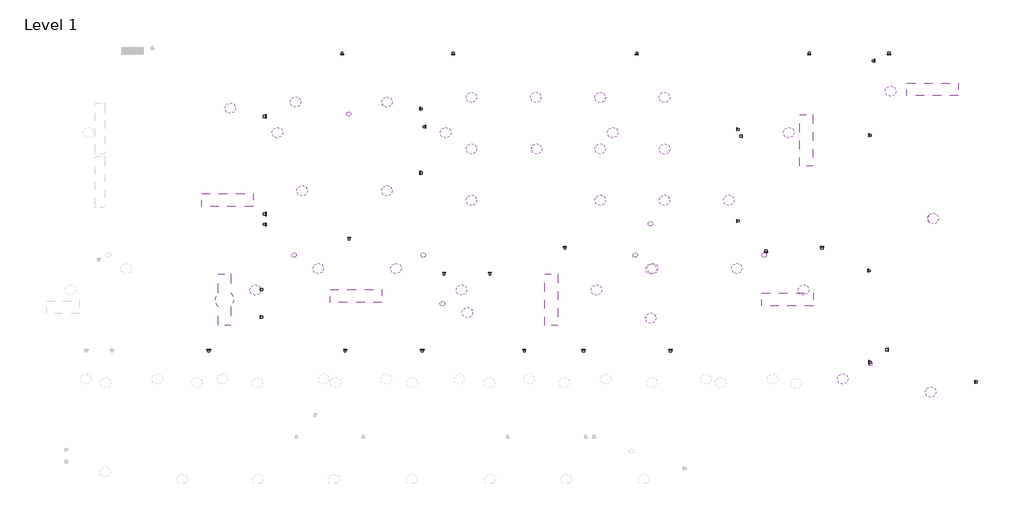
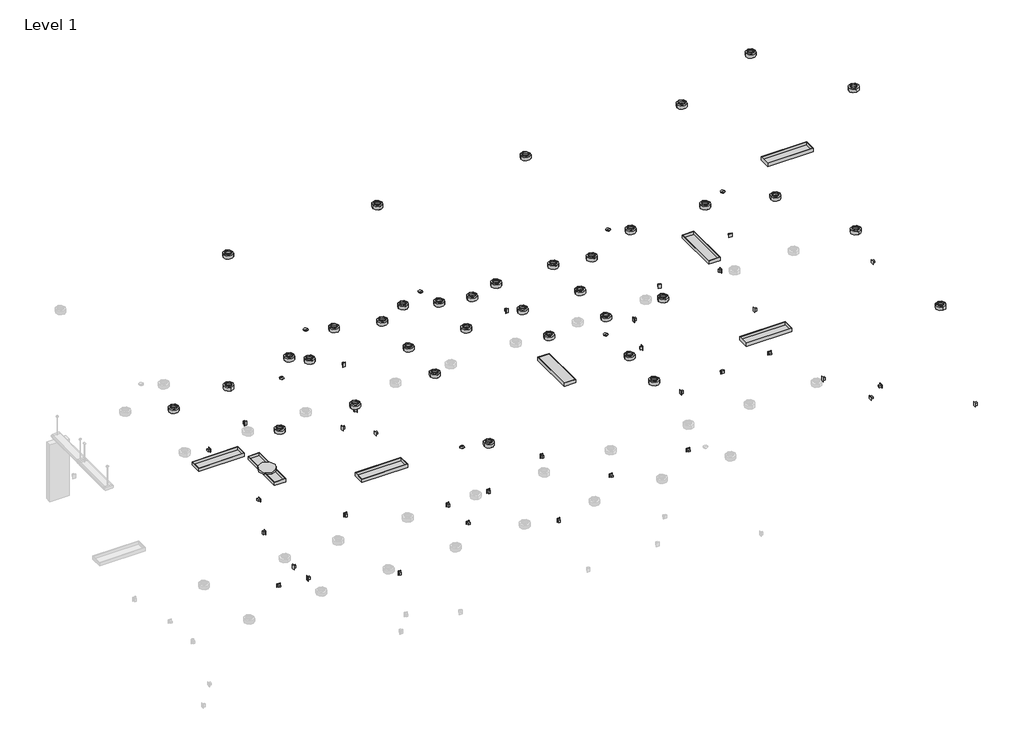
# One storey, part 3 of 3: 43 light fixtures, 22 proxies, 20 switching devices.
"""IFC4 building model written with IfcOpenShell, lengths in millimetres."""

import ifcopenshell
import ifcopenshell.guid

model = None  # the IFC model being written
_history = None  # IfcOwnerHistory: only IFC2X3 demands one
_inside = {}  # id of a spatial element -> (the spatial element, [elements in it])
_under = {}  # id of a project, library or spatial element -> (it, [spatial elements below it])
_declared = {}  # id of a project -> (the project, [libraries it declares])
_typed = {}  # id of a type object -> (the type object, [elements of that type])
_made_of = {}  # id of a material, layer set ... -> (it, [elements and type objects made of it])


def new_model(schema):
    """Start an empty IFC model of exactly this schema.

    Asked for "IFC4X3", IfcOpenShell would pick the latest addendum, in which some entities
    have other attributes; the version numbers below select the first issue.
    IFC2X3 requires an IfcOwnerHistory on every rooted entity: one is made here for all.
    """
    global model, _history
    if schema == "IFC4X3":
        model = ifcopenshell.file(schema_version=(4, 3, 0, 0))
    else:
        model = ifcopenshell.file(schema=schema)
    _inside.clear()
    _under.clear()
    _declared.clear()
    _typed.clear()
    _made_of.clear()
    _history = None
    if model.schema == "IFC2X3":
        org = make("IfcOrganization", Name="unknown")
        user = make(
            "IfcPersonAndOrganization",
            ThePerson=make("IfcPerson", FamilyName="unknown"),
            TheOrganization=org,
        )
        app = make(
            "IfcApplication",
            ApplicationDeveloper=org,
            Version="unknown",
            ApplicationFullName="unknown",
            ApplicationIdentifier="unknown",
        )
        _history = make(
            "IfcOwnerHistory",
            OwningUser=user,
            OwningApplication=app,
            ChangeAction="ADDED",
            CreationDate=0,
        )
    return model


def make(cls, **values):
    """One entity of the class cls with the attributes given. An attribute that is None is left unset."""
    return model.create_entity(
        cls, **{name: value for name, value in values.items() if value is not None}
    )


def rooted(cls, **values):
    """An entity with a GlobalId (a new one), such as an element, a storey or a relation."""
    return make(cls, GlobalId=ifcopenshell.guid.new(), OwnerHistory=_history, **values)


def si_unit(unit_type, name, prefix=None):
    """IfcSIUnit, for example si_unit("LENGTHUNIT", "METRE", prefix="MILLI")."""
    return make("IfcSIUnit", UnitType=unit_type, Prefix=prefix, Name=name)


def assignment(units):
    """IfcUnitAssignment: the units of a project."""
    return None if units is None else make("IfcUnitAssignment", Units=units)


def point(xyz):
    """IfcCartesianPoint."""
    return None if xyz is None else make("IfcCartesianPoint", Coordinates=xyz)


def direction(xyz):
    """IfcDirection."""
    return None if xyz is None else make("IfcDirection", DirectionRatios=xyz)


def frame(location, z_axis=None, x_axis=None):
    """IfcAxis2Placement3D, a coordinate frame: its origin and axes. An axis left out is left unset."""
    return make(
        "IfcAxis2Placement3D",
        Location=point(location),
        Axis=direction(z_axis),
        RefDirection=direction(x_axis),
    )


def frame_2d(location, x_axis=None):
    """IfcAxis2Placement2D, a coordinate frame in the plane: its origin and x axis."""
    return make(
        "IfcAxis2Placement2D", Location=point(location), RefDirection=direction(x_axis)
    )


def origin():
    """The frame at (0, 0, 0) with its axes left unset."""
    return frame((0.0, 0.0, 0.0))


def origin_with_axes():
    """The frame at (0, 0, 0) with the z axis (0, 0, 1) and the x axis (1, 0, 0) written out."""
    return frame((0.0, 0.0, 0.0), z_axis=(0.0, 0.0, 1.0), x_axis=(1.0, 0.0, 0.0))


def origin_2d():
    """The frame at (0, 0) in the plane with its x axis left unset."""
    return frame_2d((0.0, 0.0))


def place(relative_to, where):
    """IfcLocalPlacement: puts the frame where relative to a parent placement (None: the world)."""
    return make(
        "IfcLocalPlacement", PlacementRelTo=relative_to, RelativePlacement=where
    )


def context(
    kind, dimensions, precision=None, world=None, true_north=None, identifier=None
):
    """IfcGeometricRepresentationContext, for example the 3D "Model" context."""
    return make(
        "IfcGeometricRepresentationContext",
        ContextIdentifier=identifier,
        ContextType=kind,
        CoordinateSpaceDimension=dimensions,
        Precision=precision,
        WorldCoordinateSystem=world,
        TrueNorth=true_north,
    )


def project(units=None, contexts=None):
    """IfcProject with its units and contexts."""
    return rooted(
        "IfcProject",
        Name="project",
        RepresentationContexts=contexts,
        UnitsInContext=assignment(units),
    )


def spatial(cls, under=None, at=None, **own):
    """A site, building, storey or space (cls), placed at a placement, below another one or the project."""
    s = rooted(cls, ObjectPlacement=at, **own)
    if under is not None:
        _under.setdefault(under.id(), (under, []))[1].append(s)
    return s


def polyline(points):
    """IfcPolyline through the points."""
    return make("IfcPolyline", Points=[point(p) for p in points])


def circle_curve(where, radius):
    """IfcCircle in the frame where."""
    return make("IfcCircle", Position=where, Radius=radius)


def ellipse_curve(where, semi_axis1, semi_axis2):
    """IfcEllipse in the frame where."""
    return make(
        "IfcEllipse", Position=where, SemiAxis1=semi_axis1, SemiAxis2=semi_axis2
    )


def trimmed(basis, trim1, trim2, sense, master):
    """IfcTrimmedCurve: the piece of a basis curve between two trims."""
    return make(
        "IfcTrimmedCurve",
        BasisCurve=basis,
        Trim1=trim1,
        Trim2=trim2,
        SenseAgreement=sense,
        MasterRepresentation=master,
    )


def segment(curve, same_sense, transition):
    """IfcCompositeCurveSegment."""
    return make(
        "IfcCompositeCurveSegment",
        Transition=transition,
        SameSense=same_sense,
        ParentCurve=curve,
    )


def composite_curve(segments, self_intersect=None):
    """IfcCompositeCurve: segments joined end to end."""
    return make("IfcCompositeCurve", Segments=segments, SelfIntersect=self_intersect)


def outline(outer, holes=None, kind="AREA"):
    """IfcArbitraryClosedProfileDef: a profile drawn as a closed curve; with holes, ...WithVoids."""
    if holes is None:
        return make("IfcArbitraryClosedProfileDef", ProfileType=kind, OuterCurve=outer)
    return make(
        "IfcArbitraryProfileDefWithVoids",
        ProfileType=kind,
        OuterCurve=outer,
        InnerCurves=holes,
    )


def extrude(swept, where, along, depth):
    """IfcExtrudedAreaSolid: the profile swept, set in the frame where, extruded along a direction by depth."""
    return make(
        "IfcExtrudedAreaSolid",
        SweptArea=swept,
        Position=where,
        ExtrudedDirection=direction(along),
        Depth=depth,
    )


def shape(context_of_items, identifier, shape_type, items):
    """IfcShapeRepresentation: the items that make up one representation, for example the "Body"."""
    return make(
        "IfcShapeRepresentation",
        ContextOfItems=context_of_items,
        RepresentationIdentifier=identifier,
        RepresentationType=shape_type,
        Items=items,
    )


def source(mapping_origin, context_of_items, identifier, shape_type, items):
    """IfcRepresentationMap: a shape defined once, which mapped items show again and again."""
    return make(
        "IfcRepresentationMap",
        MappingOrigin=mapping_origin,
        MappedRepresentation=shape(context_of_items, identifier, shape_type, items),
    )


def transform(
    local_origin,
    x_axis=None,
    y_axis=None,
    z_axis=None,
    scale=None,
    scale2=None,
    scale3=None,
    uniform=True,
):
    """IfcCartesianTransformationOperator3D, or its non-uniform kind. x_axis, y_axis, z_axis: its Axis1, 2, 3."""
    if uniform:
        return make(
            "IfcCartesianTransformationOperator3D",
            Axis1=direction(x_axis),
            Axis2=direction(y_axis),
            LocalOrigin=point(local_origin),
            Scale=scale,
            Axis3=direction(z_axis),
        )
    return make(
        "IfcCartesianTransformationOperator3DnonUniform",
        Axis1=direction(x_axis),
        Axis2=direction(y_axis),
        LocalOrigin=point(local_origin),
        Scale=scale,
        Axis3=direction(z_axis),
        Scale2=scale2,
        Scale3=scale3,
    )


def mapped(mapping_source, mapping_target):
    """IfcMappedItem: shows the shape of a source again, moved by a transform."""
    return make(
        "IfcMappedItem", MappingSource=mapping_source, MappingTarget=mapping_target
    )


def made_of(thing, what):
    """Note that an element or type object is made of a material, layer set ...; save() writes the relation."""
    if what is not None:
        _made_of.setdefault(what.id(), (what, []))[1].append(thing)
    return thing


def element(
    cls,
    number,
    at=None,
    inside=None,
    cuts=None,
    type_object=None,
    material=None,
    context=None,
    identifier="Body",
    shape_type=None,
    held_by="IfcProductDefinitionShape",
    body=None,
    shapes=None,
    **own,
):
    """One element of the class cls, such as IfcWall. Its Tag is "e" and its number.

    at: its placement. inside: the storey or other place that contains it. cuts: it is an
    opening in that element (IfcRelVoidsElement). A single representation is given by context,
    identifier, shape_type and body (its items); several are given by shapes. held_by: the class
    of the entity that holds the representations. save() writes the other relations.
    """
    e = rooted(cls, Tag="e%d" % number, ObjectPlacement=at, **own)
    if body is not None:
        shapes = [shape(context, identifier, shape_type, body)]
    if shapes is not None:
        e.Representation = make(held_by, Representations=shapes)
    if inside is not None:
        _inside.setdefault(inside.id(), (inside, []))[1].append(e)
    if cuts is not None:
        rooted(
            "IfcRelVoidsElement", RelatingBuildingElement=cuts, RelatedOpeningElement=e
        )
    if type_object is not None:
        _typed.setdefault(type_object.id(), (type_object, []))[1].append(e)
    return made_of(e, material)


def aggregate(whole, parts):
    """IfcRelAggregates: a whole, such as a stair, and the parts it consists of."""
    return rooted("IfcRelAggregates", RelatingObject=whole, RelatedObjects=parts)


def save(model, path):
    """Write the relations noted so far, then the file.

    IfcRelAggregates (storeys below a building ...), IfcRelContainedInSpatialStructure (elements
    in a storey), IfcRelDefinesByType, IfcRelAssociatesMaterial and IfcRelDeclares: one each for
    every whole, place, type object, material and project.
    """
    for whole, parts in _under.values():
        aggregate(whole, parts)
    for where, things in _inside.values():
        rooted(
            "IfcRelContainedInSpatialStructure",
            RelatedElements=things,
            RelatingStructure=where,
        )
    for kind, things in _typed.values():
        rooted("IfcRelDefinesByType", RelatedObjects=things, RelatingType=kind)
    for what, things in _made_of.values():
        rooted("IfcRelAssociatesMaterial", RelatedObjects=things, RelatingMaterial=what)
    for by, libraries in _declared.values():
        rooted("IfcRelDeclares", RelatingContext=by, RelatedDefinitions=libraries)
    model.write(path)


def plane_surface(at):
    """IfcPlane: the flat surface through the origin of the frame at, square to its z axis."""
    return make("IfcPlane", Position=at)


def cylinder_surface(at, radius):
    """IfcCylindricalSurface: all points at the distance radius from the z axis of the frame at."""
    return make("IfcCylindricalSurface", Position=at, Radius=radius)


def revolved_surface(curve, axis_point, axis_direction):
    """IfcSurfaceOfRevolution: the curve turned about the line through axis_point along axis_direction."""
    return make(
        "IfcSurfaceOfRevolution",
        SweptCurve=make("IfcArbitraryOpenProfileDef", ProfileType="CURVE", Curve=curve),
        AxisPosition=make("IfcAxis1Placement", Location=point(axis_point), Axis=direction(axis_direction)),
    )


def advanced_brep(points, edges, surfaces, faces):
    """IfcAdvancedBrep: a solid bounded by faces that lie on surfaces and meet in shared edges.

    An edge is (start, end): straight between two places in points (the first is 0);
    or (start, end, curve); or (start, end, curve, False) where it runs against its curve.
    A face is (place in surfaces, loops), or (place, loops, False) where it looks against
    its surface's normal. A loop lists edges by number (the first is 1), with a minus sign
    where the edge is run from its end to its start. The first loop is the outer one.
    """
    corners = [point(p) for p in points]
    vertices = [make("IfcVertexPoint", VertexGeometry=c) for c in corners]
    made = []
    for start, end, *more in edges:
        made.append(
            make(
                "IfcEdgeCurve",
                EdgeStart=vertices[start],
                EdgeEnd=vertices[end],
                EdgeGeometry=more[0] if more else make("IfcPolyline", Points=[corners[start], corners[end]]),
                SameSense=more[1] if len(more) > 1 else True,
            )
        )
    hull = []
    for where, loops, *sense in faces:
        bounds = []
        for j, loop in enumerate(loops):
            ring = [make("IfcOrientedEdge", EdgeElement=made[abs(k) - 1], Orientation=k > 0) for k in loop]
            bounds.append(
                make(
                    "IfcFaceOuterBound" if j == 0 else "IfcFaceBound",
                    Bound=make("IfcEdgeLoop", EdgeList=ring),
                    Orientation=True,
                )
            )
        hull.append(make("IfcAdvancedFace", Bounds=bounds, FaceSurface=surfaces[where], SameSense=sense[0] if sense else True))
    return make("IfcAdvancedBrep", Outer=make("IfcClosedShell", CfsFaces=hull))


def m_duplex_receptacle_top_switched_standard_10251bba(model_context):
    return source(origin(), model_context, "Body", "SweptSolid", [
        extrude(outline(polyline([(19.05, 38.1), (19.05, -38.1), (-19.05, -38.1), (-19.05, 38.1), (19.05, 38.1)])), frame((0.0, 0.0, -53.975), z_axis=(0.0, 0.0, 1.0), x_axis=(1.0, 0.0, 0.0)), (0.0, 0.0, 1.0), 53.975),
        extrude(outline(polyline([(34.925, 57.15), (34.925, -57.15), (-34.925, -57.15), (-34.925, 57.15), (34.925, 57.15)])), origin_with_axes(), (0.0, 0.0, 1.0), 4.7625),
    ])


def light_fixture_300x1200mm_1_lamp_230v_5a723bfd(model_context):
    return source(origin(), model_context, "Body", "SweptSolid", [
        extrude(outline(composite_curve([segment(trimmed(circle_curve(frame_2d((0.0, -150.0)), 220.0), [point((-220.0, -150.0))], [point((220.0, -150.0))], False, "CARTESIAN"), True, "CONTINUOUS"), segment(trimmed(circle_curve(frame_2d((0.0, -150.0)), 220.0), [point((220.0, -150.0))], [point((-220.0, -150.0))], False, "CARTESIAN"), True, "CONTINUOUS")], self_intersect=False)), origin_with_axes(), (0.0, 0.0, 1.0), 50.8),
        extrude(outline(polyline([(587.3, -12.7), (587.3, -287.3), (-587.3, -287.3), (-587.3, -12.7), (587.3, -12.7)])), frame((0.0, 0.0, 76.2), z_axis=(0.0, 0.0, 1.0), x_axis=(1.0, 0.0, 0.0)), (0.0, 0.0, 1.0), 6.35),
        extrude(outline(polyline([(600.0, 0.0), (600.0, -300.0), (-600.0, -300.0), (-600.0, 0.0), (600.0, 0.0)]), holes=[polyline([(587.3, -12.7), (-587.3, -12.7), (-587.3, -287.3), (587.3, -287.3), (587.3, -12.7)])]), origin_with_axes(), (0.0, 0.0, 1.0), 88.9),
    ])


def ceiling_light_linear_box_300x1200_0300x1200mm_1_lamp_230v_9b76a469(model_context):
    return source(origin(), model_context, "Body", "SweptSolid", [
        extrude(outline(polyline([(587.3, -12.7), (587.3, -287.3), (-587.3, -287.3), (-587.3, -12.7), (587.3, -12.7)])), frame((0.0, 0.0, 76.2), z_axis=(0.0, 0.0, 1.0), x_axis=(1.0, 0.0, 0.0)), (0.0, 0.0, 1.0), 6.35),
        extrude(outline(polyline([(600.0, 0.0), (600.0, -300.0), (-600.0, -300.0), (-600.0, 0.0), (600.0, 0.0)]), holes=[polyline([(587.3, -12.7), (-587.3, -12.7), (-587.3, -287.3), (587.3, -287.3), (587.3, -12.7)])]), origin_with_axes(), (0.0, 0.0, 1.0), 88.9),
    ])


def ceilinglight_roundemergency_100w_230v_36b39b3f(model_context):
    return source(origin(), model_context, "Body", "SolidModel", [
        extrude(outline(composite_curve([segment(trimmed(circle_curve(origin_2d(), 82.55), [point((-82.55, 0.0))], [point((82.55, 0.0))], False, "CARTESIAN"), True, "CONTINUOUS"), segment(trimmed(circle_curve(origin_2d(), 82.55), [point((82.55, 0.0))], [point((-82.55, 0.0))], False, "CARTESIAN"), True, "CONTINUOUS")], self_intersect=False), holes=[composite_curve([segment(trimmed(circle_curve(origin_2d(), 76.2), [point((-76.2, 0.0))], [point((76.2, 0.0))], True, "CARTESIAN"), True, "CONTINUOUS"), segment(trimmed(circle_curve(origin_2d(), 76.2), [point((76.2, 0.0))], [point((-76.2, 0.0))], True, "CARTESIAN"), True, "CONTINUOUS")], self_intersect=False)]), frame((0.0, 0.0, -101.810254), z_axis=(0.0, 0.0, 1.0), x_axis=(1.0, 0.0, 0.0)), (0.0, 0.0, 1.0), 25.0),
        advanced_brep(
        [(127.0, 0.0, -74.6), (-127.0, 0.0, -74.6), (-127.0, 0.0, 14.3), (127.0, 0.0, 14.3), (76.2, 0.0, -74.6), (-76.2, 0.0, -74.6), (76.2, 0.0, -100.0), (-76.2, 0.0, -100.0), (73.025, 0.0, -100.0), (-73.025, 0.0, -100.0), (73.025, 0.0, -71.425), (-73.025, 0.0, -71.425), (123.825, 0.0, -71.425), (-123.825, 0.0, -71.425), (123.825, 0.0, 11.125), (-123.825, 0.0, 11.125), (0.0, 0.0, 11.125), (0.0, 0.0, 14.3)],
        [
            (0, 1, circle_curve(frame((0.0, 0.0, -74.6), z_axis=(0.0, 0.0, 1.0), x_axis=(-1.0, 0.0, 0.0)), 127.0)),
            (1, 2),
            (2, 3, circle_curve(frame((0.0, 0.0, 14.3), z_axis=(0.0, 0.0, -1.0), x_axis=(-1.0, 0.0, 0.0)), 127.0)),
            (3, 0),
            (1, 0, circle_curve(frame((0.0, 0.0, -74.6), z_axis=(0.0, 0.0, 1.0), x_axis=(-1.0, 0.0, 0.0)), 127.0)),
            (3, 2, circle_curve(frame((0.0, 0.0, 14.3), z_axis=(0.0, 0.0, -1.0), x_axis=(-1.0, 0.0, 0.0)), 127.0)),
            (4, 5, circle_curve(frame((0.0, 0.0, -74.6), z_axis=(0.0, 0.0, 1.0), x_axis=(-1.0, 0.0, 0.0)), 76.2)),
            (5, 1),
            (0, 4),
            (5, 4, circle_curve(frame((0.0, 0.0, -74.6), z_axis=(0.0, 0.0, 1.0), x_axis=(-1.0, 0.0, 0.0)), 76.2)),
            (6, 7, circle_curve(frame((0.0, 0.0, -100.0), z_axis=(0.0, 0.0, 1.0), x_axis=(-1.0, 0.0, 0.0)), 76.2)),
            (7, 5),
            (4, 6),
            (7, 6, circle_curve(frame((0.0, 0.0, -100.0), z_axis=(0.0, 0.0, 1.0), x_axis=(-1.0, 0.0, 0.0)), 76.2)),
            (8, 9, circle_curve(frame((0.0, 0.0, -100.0), z_axis=(0.0, 0.0, 1.0), x_axis=(-1.0, 0.0, 0.0)), 73.025)),
            (9, 7),
            (6, 8),
            (9, 8, circle_curve(frame((0.0, 0.0, -100.0), z_axis=(0.0, 0.0, 1.0), x_axis=(-1.0, 0.0, 0.0)), 73.025)),
            (10, 11, circle_curve(frame((0.0, 0.0, -71.425), z_axis=(0.0, 0.0, 1.0), x_axis=(-1.0, 0.0, 0.0)), 73.025)),
            (11, 9),
            (8, 10),
            (11, 10, circle_curve(frame((0.0, 0.0, -71.425), z_axis=(0.0, 0.0, 1.0), x_axis=(-1.0, 0.0, 0.0)), 73.025)),
            (12, 13, circle_curve(frame((0.0, 0.0, -71.425), z_axis=(0.0, 0.0, 1.0), x_axis=(-1.0, 0.0, 0.0)), 123.825)),
            (13, 11),
            (10, 12),
            (13, 12, circle_curve(frame((0.0, 0.0, -71.425), z_axis=(0.0, 0.0, 1.0), x_axis=(-1.0, 0.0, 0.0)), 123.825)),
            (14, 15, circle_curve(frame((0.0, 0.0, 11.125), z_axis=(0.0, 0.0, 1.0), x_axis=(-1.0, 0.0, 0.0)), 123.825)),
            (15, 13),
            (12, 14),
            (15, 14, circle_curve(frame((0.0, 0.0, 11.125), z_axis=(0.0, 0.0, 1.0), x_axis=(-1.0, 0.0, 0.0)), 123.825)),
            (16, 15),
            (14, 16),
            (2, 17),
            (17, 3),
        ],
        [
            cylinder_surface(frame((0.0, 0.0, 11.125), z_axis=(0.0, 0.0, -1.0), x_axis=(-1.0, 0.0, 0.0)), 127.0),
            plane_surface(frame((0.0, 0.0, -74.6), z_axis=(0.0, 0.0, -1.0), x_axis=(-1.0, 0.0, 0.0))),
            cylinder_surface(frame((0.0, 0.0, 11.125), z_axis=(0.0, 0.0, -1.0), x_axis=(-1.0, 0.0, 0.0)), 76.2),
            plane_surface(frame((0.0, 0.0, -100.0), z_axis=(0.0, 0.0, -1.0), x_axis=(-1.0, 0.0, 0.0))),
            revolved_surface(polyline([(-73.025, 0.0, -100.0), (-73.025, 0.0, -71.425)]), (0.0, 0.0, 11.125), (0.0, 0.0, -1.0)),
            plane_surface(frame((0.0, 0.0, -71.425), z_axis=(0.0, 0.0, 1.0), x_axis=(-1.0, 0.0, 0.0))),
            revolved_surface(polyline([(-123.825, 0.0, -71.425), (-123.825, 0.0, 11.125)]), (0.0, 0.0, 11.125), (0.0, 0.0, -1.0)),
            plane_surface(frame((0.0, 0.0, 11.125), z_axis=(0.0, 0.0, -1.0), x_axis=(-1.0, 0.0, 0.0))),
            plane_surface(frame((0.0, 0.0, 14.3), z_axis=(0.0, 0.0, 1.0), x_axis=(-1.0, 0.0, 0.0))),
        ],
        [
            (0, [[1, 2, 3, 4]]),
            (0, [[5, -4, 6, -2]]),
            (1, [[7, 8, -1, 9]]),
            (1, [[10, -9, -5, -8]]),
            (2, [[11, 12, -7, 13]]),
            (2, [[14, -13, -10, -12]]),
            (3, [[15, 16, -11, 17]]),
            (3, [[18, -17, -14, -16]]),
            (4, [[19, 20, -15, 21]]),
            (4, [[22, -21, -18, -20]]),
            (5, [[23, 24, -19, 25]]),
            (5, [[26, -25, -22, -24]]),
            (6, [[27, 28, -23, 29]]),
            (6, [[30, -29, -26, -28]]),
            (7, [[31, -27, 32]]),
            (7, [[-32, -30, -31]]),
            (8, [[-3, 33, 34]]),
            (8, [[-6, -34, -33]]),
        ],
    ),
    ])


def ceilingoccupancysensor_450_02cbfb90(model_context):
    return source(origin(), model_context, "Body", "AdvancedBrep", [
        advanced_brep(
        [(-12.7998992, 0.0, 32.54375), (12.7998992, 0.0, 32.54375), (0.0, 0.0, 35.5203125), (-19.3725919, 0.0, 32.54375), (19.3725919, 0.0, 32.54375), (-21.6519708, 0.0, 28.5957499), (21.6519708, 0.0, 28.5957499), (-27.834758, 0.0, 28.5957499), (27.834758, 0.0, 28.5957499), (-57.15, 0.0, 2.3911967), (57.15, 0.0, 2.3911967), (-56.5092808, 0.0, 0.0), (56.5092808, 0.0, 0.0), (0.0, 0.0, 0.0)],
        [
            (0, 1, circle_curve(frame((0.0, 0.0, 32.54375), z_axis=(0.0, 0.0, 1.0), x_axis=(1.0, 0.0, 0.0)), 12.7998992)),
            (1, 2, circle_curve(frame((0.750087, 0.0, 9.7363307), z_axis=(0.0, -1.0, 0.0), x_axis=(1.0, 0.0, 0.0)), 25.79489)),
            (2, 0, circle_curve(frame((-0.750087, 0.0, 9.7363307), z_axis=(0.0, -1.0, 0.0), x_axis=(-1.0, 0.0, 0.0)), 25.79489)),
            (1, 0, circle_curve(frame((0.0, 0.0, 32.54375), z_axis=(0.0, 0.0, 1.0), x_axis=(1.0, 0.0, 0.0)), 12.7998992)),
            (3, 4, circle_curve(frame((0.0, 0.0, 32.54375), z_axis=(0.0, 0.0, 1.0), x_axis=(1.0, 0.0, 0.0)), 19.3725919)),
            (4, 1),
            (0, 3),
            (4, 3, circle_curve(frame((0.0, 0.0, 32.54375), z_axis=(0.0, 0.0, 1.0), x_axis=(1.0, 0.0, 0.0)), 19.3725919)),
            (5, 6, circle_curve(frame((0.0, 0.0, 28.5957499), z_axis=(0.0, 0.0, 1.0), x_axis=(1.0, 0.0, 0.0)), 21.6519708)),
            (6, 4),
            (3, 5),
            (6, 5, circle_curve(frame((0.0, 0.0, 28.5957499), z_axis=(0.0, 0.0, 1.0), x_axis=(1.0, 0.0, 0.0)), 21.6519708)),
            (7, 8, circle_curve(frame((0.0, 0.0, 28.5957499), z_axis=(0.0, 0.0, 1.0), x_axis=(1.0, 0.0, 0.0)), 27.834758)),
            (8, 6),
            (5, 7),
            (8, 7, circle_curve(frame((0.0, 0.0, 28.5957499), z_axis=(0.0, 0.0, 1.0), x_axis=(1.0, 0.0, 0.0)), 27.834758)),
            (9, 10, circle_curve(frame((0.0, 0.0, 2.3911967), z_axis=(0.0, 0.0, 1.0), x_axis=(1.0, 0.0, 0.0)), 57.15)),
            (10, 8, circle_curve(frame((20.1846327, 0.0, -9.4623798), z_axis=(0.0, -1.0, 0.0), x_axis=(1.0, 0.0, 0.0)), 38.8193979)),
            (7, 9, circle_curve(frame((-20.1846327, 0.0, -9.4623798), z_axis=(0.0, -1.0, 0.0), x_axis=(-1.0, 0.0, 0.0)), 38.8193979)),
            (10, 9, circle_curve(frame((0.0, 0.0, 2.3911967), z_axis=(0.0, 0.0, 1.0), x_axis=(1.0, 0.0, 0.0)), 57.15)),
            (11, 12, circle_curve(origin_with_axes(), 56.5092808)),
            (12, 10),
            (9, 11),
            (12, 11, circle_curve(origin_with_axes(), 56.5092808)),
            (13, 12),
            (11, 13),
        ],
        [
            revolved_surface(trimmed(ellipse_curve(frame((0.750087, 0.0, 9.7363307), z_axis=(0.0, 1.0, 0.0), x_axis=(1.0, 0.0, 0.0)), 25.79489, 25.79489), [point((0.0, 0.0, 35.5203125))], [point((12.7998992, 0.0, 32.54375))], True, "CARTESIAN"), (0.0, 0.0, 38.1), (0.0, 0.0, -1.0)),
            plane_surface(frame((0.0, 0.0, 32.54375), z_axis=(0.0, 0.0, 1.0), x_axis=(1.0, 0.0, 0.0))),
            revolved_surface(polyline([(19.3725919, 0.0, 32.54375), (21.6519708, 0.0, 28.5957499)]), (0.0, 0.0, 38.1), (0.0, 0.0, -1.0)),
            plane_surface(frame((0.0, 0.0, 28.5957499), z_axis=(0.0, 0.0, 1.0), x_axis=(1.0, 0.0, 0.0))),
            revolved_surface(trimmed(ellipse_curve(frame((20.1846327, 0.0, -9.4623798), z_axis=(0.0, 1.0, 0.0), x_axis=(1.0, 0.0, 0.0)), 38.8193979, 38.8193979), [point((27.834758, 0.0, 28.5957499))], [point((57.15, 0.0, 2.3911967))], True, "CARTESIAN"), (0.0, 0.0, 38.1), (0.0, 0.0, -1.0)),
            revolved_surface(polyline([(57.15, 0.0, 2.3911967), (56.5092808, 0.0, 0.0)]), (0.0, 0.0, 38.1), (0.0, 0.0, -1.0)),
            plane_surface(frame((0.0, 0.0, 0.0), z_axis=(0.0, 0.0, -1.0), x_axis=(1.0, 0.0, 0.0))),
        ],
        [
            (0, [[1, 2, 3]]),
            (0, [[4, -3, -2]]),
            (1, [[5, 6, -1, 7]]),
            (1, [[8, -7, -4, -6]]),
            (2, [[9, 10, -5, 11]]),
            (2, [[12, -11, -8, -10]]),
            (3, [[13, 14, -9, 15]]),
            (3, [[16, -15, -12, -14]]),
            (4, [[17, 18, -13, 19]]),
            (4, [[20, -19, -16, -18]]),
            (5, [[21, 22, -17, 23]]),
            (5, [[24, -23, -20, -22]]),
            (6, [[25, -21, 26]]),
            (6, [[-26, -24, -25]]),
        ],
    ),
    ])


def lighting_switches_four_way_four_way_switch_ab144c04(model_context):
    return source(origin(), model_context, "Body", "SweptSolid", [
        extrude(outline(polyline([(43.0, -86.0), (-43.0, -86.0), (-43.0, 0.0), (43.0, 0.0), (43.0, -86.0)])), origin_with_axes(), (0.0, 0.0, 1.0), 5.0),
        extrude(outline(polyline([(27.0, -67.0), (-27.0, -67.0), (-27.0, -19.0), (27.0, -19.0), (27.0, -67.0)])), frame((0.0, 0.0, -54.0), z_axis=(0.0, 0.0, 1.0), x_axis=(1.0, 0.0, 0.0)), (0.0, 0.0, 1.0), 54.0),
    ])


model = new_model("IFC4")

# Units and contexts
model_context = context("Model", 3, world=origin())
ifc_project = project(units=[si_unit("LENGTHUNIT", "METRE", prefix="MILLI")], contexts=[model_context])

# Site, building, storey
site = spatial("IfcSite", under=ifc_project)
building = spatial("IfcBuilding", under=site)
storey = spatial("IfcBuildingStorey", under=building, Name="Level 1", Elevation=100000.0)

# Proxies
placement = place(None, origin())
m_duplex_receptacle_top_switched_standard_shape = m_duplex_receptacle_top_switched_standard_10251bba(model_context)
element("IfcBuildingElementProxy", 1, Name="M_Duplex Receptacle OFCI : GFCI", ObjectType="M_Duplex Receptacle OFCI : GFCI", at=placement, inside=storey, context=model_context, shape_type="MappedRepresentation", body=[
    mapped(m_duplex_receptacle_top_switched_standard_shape, transform((21875.68, 13410.0390001, 101112.2), x_axis=(0.0, 1.0, 0.0), y_axis=(0.0, 0.0, 1.0), z_axis=(1.0, 0.0, 0.0))),
])
element("IfcBuildingElementProxy", 2, Name="M_Duplex Receptacle OFCI : GFCI", ObjectType="M_Duplex Receptacle OFCI : GFCI", at=placement, inside=storey, context=model_context, shape_type="MappedRepresentation", body=[
    mapped(m_duplex_receptacle_top_switched_standard_shape, transform((22524.0144082, 15100.039, 101112.15), x_axis=(1.0, 0.0, 0.0), y_axis=(0.0, 0.0, 1.0), z_axis=(0.0, -1.0, 0.0))),
])
element("IfcBuildingElementProxy", 3, Name="M_Duplex Receptacle OFCI : GFCI", ObjectType="M_Duplex Receptacle OFCI : GFCI", at=placement, inside=storey, context=model_context, shape_type="MappedRepresentation", body=[
    mapped(m_duplex_receptacle_top_switched_standard_shape, transform((26810.005, 15100.039, 101112.2), x_axis=(1.0, 0.0, 0.0), y_axis=(0.0, 0.0, 1.0), z_axis=(0.0, -1.0, 0.0))),
])
element("IfcBuildingElementProxy", 4, Name="M_Duplex Receptacle OFCI : GFCI", ObjectType="M_Duplex Receptacle OFCI : GFCI", at=placement, inside=storey, context=model_context, shape_type="MappedRepresentation", body=[
    mapped(m_duplex_receptacle_top_switched_standard_shape, transform((29138.905, 13350.0390001, 101112.2), x_axis=(0.0, -1.0, 0.0), y_axis=(0.0, 0.0, 1.0), z_axis=(-1.0, 0.0, 0.0))),
])
element("IfcBuildingElementProxy", 5, Name="M_Receptacle - 220V : Standard", ObjectType="M_Receptacle - 220V : Standard", at=placement, inside=storey, context=model_context, shape_type="MappedRepresentation", body=[
    mapped(m_duplex_receptacle_top_switched_standard_shape, transform((20000.005, 8200.039, 100390.0), x_axis=(-1.0, 0.0, 0.0), y_axis=(0.0, 0.0, 1.0), z_axis=(0.0, 1.0, 0.0))),
])
element("IfcBuildingElementProxy", 6, Name="M_Receptacle - 220V : Standard", ObjectType="M_Receptacle - 220V : Standard", at=placement, inside=storey, context=model_context, shape_type="MappedRepresentation", body=[
    mapped(m_duplex_receptacle_top_switched_standard_shape, transform((20092.5944791, 10823.4147145, 100390.0), x_axis=(-1.0, 0.0, 0.0), y_axis=(0.0, 0.0, 1.0), z_axis=(0.0, 1.0, 0.0))),
])
element("IfcBuildingElementProxy", 7, Name="M_Receptacle - 220V : Standard", ObjectType="M_Receptacle - 220V : Standard", at=placement, inside=storey, context=model_context, shape_type="MappedRepresentation", body=[
    mapped(m_duplex_receptacle_top_switched_standard_shape, transform((21750.68, 13830.0390001, 100390.0), x_axis=(0.0, -1.0, 0.0), y_axis=(0.0, 0.0, 1.0), z_axis=(-1.0, 0.0, 0.0))),
])
element("IfcBuildingElementProxy", 8, Name="M_Receptacle - 220V : Standard", ObjectType="M_Receptacle - 220V : Standard", at=placement, inside=storey, context=model_context, shape_type="MappedRepresentation", body=[
    mapped(m_duplex_receptacle_top_switched_standard_shape, transform((19929.5065734, 15100.039, 100390.0), x_axis=(1.0, 0.0, 0.0), y_axis=(0.0, 0.0, 1.0), z_axis=(0.0, -1.0, 0.0))),
])
element("IfcBuildingElementProxy", 9, Name="M_Receptacle - 220V : Standard", ObjectType="M_Receptacle - 220V : Standard", at=placement, inside=storey, context=model_context, shape_type="MappedRepresentation", body=[
    mapped(m_duplex_receptacle_top_switched_standard_shape, transform((18149.8175, 11130.039, 100390.0), x_axis=(0.0, 1.0, 0.0), y_axis=(0.0, 0.0, 1.0), z_axis=(1.0, 0.0, 0.0))),
])
element("IfcBuildingElementProxy", 10, Name="M_Receptacle - 220V : Standard", ObjectType="M_Receptacle - 220V : Standard", at=placement, inside=storey, context=model_context, shape_type="MappedRepresentation", body=[
    mapped(m_duplex_receptacle_top_switched_standard_shape, transform((25130.005, 10605.039, 100390.0), x_axis=(-1.0, 0.0, 0.0), y_axis=(0.0, 0.0, 1.0), z_axis=(0.0, 1.0, 0.0))),
])
element("IfcBuildingElementProxy", 11, Name="M_Receptacle - 220V : Standard", ObjectType="M_Receptacle - 220V : Standard", at=placement, inside=storey, context=model_context, shape_type="MappedRepresentation", body=[
    mapped(m_duplex_receptacle_top_switched_standard_shape, transform((29138.905, 11210.0390001, 100390.0), x_axis=(0.0, -1.0, 0.0), y_axis=(0.0, 0.0, 1.0), z_axis=(-1.0, 0.0, 0.0))),
])
element("IfcBuildingElementProxy", 12, Name="M_Receptacle - 220V : Standard", ObjectType="M_Receptacle - 220V : Standard", at=placement, inside=storey, context=model_context, shape_type="MappedRepresentation", body=[
    mapped(m_duplex_receptacle_top_switched_standard_shape, transform((32225.005, 13210.0390001, 100390.0), x_axis=(0.0, -1.0, 0.0), y_axis=(0.0, 0.0, 1.0), z_axis=(-1.0, 0.0, 0.0))),
])
element("IfcBuildingElementProxy", 13, Name="M_Receptacle - 220V : Standard", ObjectType="M_Receptacle - 220V : Standard", at=placement, inside=storey, context=model_context, shape_type="MappedRepresentation", body=[
    mapped(m_duplex_receptacle_top_switched_standard_shape, transform((29263.905, 13190.0390001, 100390.0), x_axis=(0.0, 1.0, 0.0), y_axis=(0.0, 0.0, 1.0), z_axis=(1.0, 0.0, 0.0))),
])
element("IfcBuildingElementProxy", 14, Name="M_Receptacle - 220V : Standard", ObjectType="M_Receptacle - 220V : Standard", at=placement, inside=storey, context=model_context, shape_type="MappedRepresentation", body=[
    mapped(m_duplex_receptacle_top_switched_standard_shape, transform((30830.005, 15100.039, 100390.0), x_axis=(1.0, 0.0, 0.0), y_axis=(0.0, 0.0, 1.0), z_axis=(0.0, -1.0, 0.0))),
])
element("IfcBuildingElementProxy", 15, Name="M_Receptacle - 220V : Standard", ObjectType="M_Receptacle - 220V : Standard", at=placement, inside=storey, context=model_context, shape_type="MappedRepresentation", body=[
    mapped(m_duplex_receptacle_top_switched_standard_shape, transform((32350.005, 14950.039, 100390.0), x_axis=(0.0, 1.0, 0.0), y_axis=(0.0, 0.0, 1.0), z_axis=(1.0, 0.0, 0.0))),
])
element("IfcBuildingElementProxy", 16, Name="M_Receptacle - 220V : Standard", ObjectType="M_Receptacle - 220V : Standard", at=placement, inside=storey, context=model_context, shape_type="MappedRepresentation", body=[
    mapped(m_duplex_receptacle_top_switched_standard_shape, transform((34700.005, 7450.0390001, 100390.0), x_axis=(0.0, -1.0, 0.0), y_axis=(0.0, 0.0, 1.0), z_axis=(-1.0, 0.0, 0.0))),
])
element("IfcBuildingElementProxy", 17, Name="M_Receptacle - 220V : Standard", ObjectType="M_Receptacle - 220V : Standard", at=placement, inside=storey, context=model_context, shape_type="MappedRepresentation", body=[
    mapped(m_duplex_receptacle_top_switched_standard_shape, transform((24185.577135, 8200.039, 100390.0), x_axis=(-1.0, 0.0, 0.0), y_axis=(0.0, 0.0, 1.0), z_axis=(0.0, 1.0, 0.0))),
])
element("IfcBuildingElementProxy", 18, Name="M_Receptacle - 220V : Standard", ObjectType="M_Receptacle - 220V : Standard", at=placement, inside=storey, context=model_context, shape_type="MappedRepresentation", body=[
    mapped(m_duplex_receptacle_top_switched_standard_shape, transform((32202.78, 10050.0390001, 100390.0), x_axis=(0.0, -1.0, 0.0), y_axis=(0.0, 0.0, 1.0), z_axis=(-1.0, 0.0, 0.0))),
])
element("IfcBuildingElementProxy", 19, Name="M_Receptacle - 220V : Standard", ObjectType="M_Receptacle - 220V : Standard", at=placement, inside=storey, context=model_context, shape_type="MappedRepresentation", body=[
    mapped(m_duplex_receptacle_top_switched_standard_shape, transform((18024.8175, 9610.0390001, 100390.0), x_axis=(0.0, -1.0, 0.0), y_axis=(0.0, 0.0, 1.0), z_axis=(-1.0, 0.0, 0.0))),
])
element("IfcBuildingElementProxy", 20, Name="M_Receptacle - 220V : Standard", ObjectType="M_Receptacle - 220V : Standard", at=placement, inside=storey, context=model_context, shape_type="MappedRepresentation", body=[
    mapped(m_duplex_receptacle_top_switched_standard_shape, transform((23377.5364464, 10002.4709645, 100390.0), x_axis=(-1.0, 0.0, 0.0), y_axis=(0.0, 0.0, 1.0), z_axis=(0.0, 1.0, 0.0))),
])
element("IfcBuildingElementProxy", 21, Name="M_Receptacle - 220V : Standard", ObjectType="M_Receptacle - 220V : Standard", at=placement, inside=storey, context=model_context, shape_type="MappedRepresentation", body=[
    mapped(m_duplex_receptacle_top_switched_standard_shape, transform((22309.5634447, 10002.4709645, 100390.0), x_axis=(-1.0, 0.0, 0.0), y_axis=(0.0, 0.0, 1.0), z_axis=(0.0, 1.0, 0.0))),
])
element("IfcBuildingElementProxy", 22, Name="M_Receptacle - DATA socket : Standard", ObjectType="M_Receptacle - DATA socket : Standard", at=placement, inside=storey, context=model_context, shape_type="MappedRepresentation", body=[
    mapped(m_duplex_receptacle_top_switched_standard_shape, transform((18024.8175, 8966.607737, 100460.0), x_axis=(0.0, -1.0, 0.0), y_axis=(0.0, 0.0, 1.0), z_axis=(-1.0, 0.0, 0.0))),
])

# Light fixtures
light_fixture_300x1200mm_1_lamp_230v_shape = light_fixture_300x1200mm_1_lamp_230v_5a723bfd(model_context)
element("IfcLightFixture", 23, ObjectType="Ceiling Light - Linear Box emergency light 300x1200mm 1Lamp 230 v : 300x1200mm(1 Lamp) - 230V", at=placement, inside=storey, context=model_context, shape_type="MappedRepresentation", body=[
    mapped(light_fixture_300x1200mm_1_lamp_230v_shape, transform((17036.2976312, 9366.5181325, 103600.0), x_axis=(0.0, -1.0, 0.0), y_axis=(-1.0, 0.0, 0.0), z_axis=(0.0, 0.0, -1.0))),
])
ceiling_light_linear_box_300x1200_0300x1200mm_1_lamp_230v_shape = ceiling_light_linear_box_300x1200_0300x1200mm_1_lamp_230v_9b76a469(model_context)
element("IfcLightFixture", 24, ObjectType="Ceiling Light - Linear Box 300x1200 : 0300x1200mm(1 Lamp) - 230V", at=placement, inside=storey, context=model_context, shape_type="MappedRepresentation", body=[
    mapped(ceiling_light_linear_box_300x1200_0300x1200mm_1_lamp_230v_shape, transform((20255.9330641, 9311.4870287, 102440.0), x_axis=(1.0, 0.0, 0.0), y_axis=(0.0, -1.0, 0.0), z_axis=(0.0, 0.0, -1.0))),
])
element("IfcLightFixture", 25, ObjectType="Ceiling Light - Linear Box 300x1200 : 0300x1200mm(1 Lamp) - 230V", at=placement, inside=storey, context=model_context, shape_type="MappedRepresentation", body=[
    mapped(ceiling_light_linear_box_300x1200_0300x1200mm_1_lamp_230v_shape, transform((30612.07484, 13086.7781336, 102750.0), x_axis=(0.0, -1.0, 0.0), y_axis=(-1.0, 0.0, 0.0), z_axis=(0.0, 0.0, -1.0))),
])
element("IfcLightFixture", 26, ObjectType="Ceiling Light - Linear Box 300x1200 : 0300x1200mm(1 Lamp) - 230V", at=placement, inside=storey, context=model_context, shape_type="MappedRepresentation", body=[
    mapped(ceiling_light_linear_box_300x1200_0300x1200mm_1_lamp_230v_shape, transform((24963.8097294, 9366.5181325, 103600.0), x_axis=(0.0, -1.0, 0.0), y_axis=(1.0, 0.0, 0.0), z_axis=(0.0, 0.0, 1.0))),
])
element("IfcLightFixture", 27, ObjectType="Ceiling Light - Linear Box 300x1200 : 0300x1200mm(1 Lamp) - 230V", at=placement, inside=storey, context=model_context, shape_type="MappedRepresentation", body=[
    mapped(ceiling_light_linear_box_300x1200_0300x1200mm_1_lamp_230v_shape, transform((30321.2991933, 9229.3597831, 102750.0), x_axis=(1.0, 0.0, 0.0), y_axis=(0.0, -1.0, 0.0), z_axis=(0.0, 0.0, -1.0))),
])
element("IfcLightFixture", 28, ObjectType="Ceiling Light - Linear Box 300x1200 : 0300x1200mm(1 Lamp) - 230V", at=placement, inside=storey, context=model_context, shape_type="MappedRepresentation", body=[
    mapped(ceiling_light_linear_box_300x1200_0300x1200mm_1_lamp_230v_shape, transform((17254.2627424, 11547.5483962, 102440.0), x_axis=(1.0, 0.0, 0.0), y_axis=(0.0, -1.0, 0.0), z_axis=(0.0, 0.0, -1.0))),
])
element("IfcLightFixture", 29, ObjectType="Ceiling Light - Linear Box 300x1200 : 0300x1200mm(1 Lamp) - 230V", at=placement, inside=storey, context=model_context, shape_type="MappedRepresentation", body=[
    mapped(ceiling_light_linear_box_300x1200_0300x1200mm_1_lamp_230v_shape, transform((33710.0000096, 14430.0000096, 103600.0), x_axis=(-1.0, 0.0, 0.0), y_axis=(0.0, 1.0, 0.0), z_axis=(0.0, 0.0, -1.0))),
])
ceilinglight_roundemergency_100w_230v_shape = ceilinglight_roundemergency_100w_230v_36b39b3f(model_context)
element("IfcLightFixture", 30, ObjectType="CeilingLight-RoundEmergency : 100W - 230V", at=placement, inside=storey, context=model_context, shape_type="MappedRepresentation", body=[
    mapped(ceilinglight_roundemergency_100w_230v_shape, transform((17318.3502465, 13844.3787201, 102440.0), x_axis=(1.0, 0.0, 0.0), y_axis=(0.0, -1.0, 0.0), z_axis=(0.0, 0.0, -1.0))),
])
element("IfcLightFixture", 31, ObjectType="CeilingLight-RoundEmergency : 100W - 230V", at=placement, inside=storey, context=model_context, shape_type="MappedRepresentation", body=[
    mapped(ceilinglight_roundemergency_100w_230v_shape, transform((18845.5635409, 13990.8003679, 102440.0), x_axis=(0.0, -1.0, 0.0), y_axis=(-1.0, 0.0, 0.0), z_axis=(0.0, 0.0, -1.0))),
])
element("IfcLightFixture", 32, ObjectType="CeilingLight-RoundEmergency : 100W - 230V", at=placement, inside=storey, context=model_context, shape_type="MappedRepresentation", body=[
    mapped(ceilinglight_roundemergency_100w_230v_shape, transform((20977.1328935, 13986.3413965, 102440.0), x_axis=(1.0, 0.0, 0.0), y_axis=(0.0, -1.0, 0.0), z_axis=(0.0, 0.0, -1.0))),
])
element("IfcLightFixture", 33, ObjectType="CeilingLight-RoundEmergency : 100W - 230V", at=placement, inside=storey, context=model_context, shape_type="MappedRepresentation", body=[
    mapped(ceilinglight_roundemergency_100w_230v_shape, transform((20976.5521018, 11915.8490177, 102440.0), x_axis=(1.0, 0.0, 0.0), y_axis=(0.0, -1.0, 0.0), z_axis=(0.0, 0.0, -1.0))),
])
element("IfcLightFixture", 34, ObjectType="CeilingLight-RoundEmergency : 100W - 230V", at=placement, inside=storey, context=model_context, shape_type="MappedRepresentation", body=[
    mapped(ceilinglight_roundemergency_100w_230v_shape, transform((18996.5521018, 11915.8490177, 102440.0), x_axis=(1.0, 0.0, 0.0), y_axis=(0.0, -1.0, 0.0), z_axis=(0.0, 0.0, -1.0))),
])
element("IfcLightFixture", 35, ObjectType="CeilingLight-RoundEmergency : 100W - 230V", at=placement, inside=storey, context=model_context, shape_type="MappedRepresentation", body=[
    mapped(ceilinglight_roundemergency_100w_230v_shape, transform((22949.2438181, 12894.4255613, 102750.0), x_axis=(1.0, 0.0, 0.0), y_axis=(0.0, -1.0, 0.0), z_axis=(0.0, 0.0, -1.0))),
])
element("IfcLightFixture", 36, ObjectType="CeilingLight-RoundEmergency : 100W - 230V", at=placement, inside=storey, context=model_context, shape_type="MappedRepresentation", body=[
    mapped(ceilinglight_roundemergency_100w_230v_shape, transform((24469.2438181, 12894.4255613, 102750.0), x_axis=(1.0, 0.0, 0.0), y_axis=(0.0, -1.0, 0.0), z_axis=(0.0, 0.0, -1.0))),
])
element("IfcLightFixture", 37, ObjectType="CeilingLight-RoundEmergency : 100W - 230V", at=placement, inside=storey, context=model_context, shape_type="MappedRepresentation", body=[
    mapped(ceilinglight_roundemergency_100w_230v_shape, transform((25949.2438181, 12894.4255613, 102750.0), x_axis=(1.0, 0.0, 0.0), y_axis=(0.0, -1.0, 0.0), z_axis=(0.0, 0.0, -1.0))),
])
element("IfcLightFixture", 38, ObjectType="CeilingLight-RoundEmergency : 100W - 230V", at=placement, inside=storey, context=model_context, shape_type="MappedRepresentation", body=[
    mapped(ceilinglight_roundemergency_100w_230v_shape, transform((27455.9396321, 12887.8217054, 102750.0), x_axis=(1.0, 0.0, 0.0), y_axis=(0.0, -1.0, 0.0), z_axis=(0.0, 0.0, -1.0))),
])
element("IfcLightFixture", 39, ObjectType="CeilingLight-RoundEmergency : 100W - 230V", at=placement, inside=storey, context=model_context, shape_type="MappedRepresentation", body=[
    mapped(ceilinglight_roundemergency_100w_230v_shape, transform((27449.2438181, 14094.4255613, 102750.0), x_axis=(1.0, 0.0, 0.0), y_axis=(0.0, -1.0, 0.0), z_axis=(0.0, 0.0, -1.0))),
])
element("IfcLightFixture", 40, ObjectType="CeilingLight-RoundEmergency : 100W - 230V", at=placement, inside=storey, context=model_context, shape_type="MappedRepresentation", body=[
    mapped(ceilinglight_roundemergency_100w_230v_shape, transform((22949.2438181, 11694.3865613, 102750.0), x_axis=(1.0, 0.0, 0.0), y_axis=(0.0, -1.0, 0.0), z_axis=(0.0, 0.0, -1.0))),
])
element("IfcLightFixture", 41, ObjectType="CeilingLight-RoundEmergency : 100W - 230V", at=placement, inside=storey, context=model_context, shape_type="MappedRepresentation", body=[
    mapped(ceilinglight_roundemergency_100w_230v_shape, transform((22949.2438181, 14094.4255613, 102750.0), x_axis=(1.0, 0.0, 0.0), y_axis=(0.0, -1.0, 0.0), z_axis=(0.0, 0.0, -1.0))),
])
element("IfcLightFixture", 42, ObjectType="CeilingLight-RoundEmergency : 100W - 230V", at=placement, inside=storey, context=model_context, shape_type="MappedRepresentation", body=[
    mapped(ceilinglight_roundemergency_100w_230v_shape, transform((24449.2438181, 14094.4255613, 102750.0), x_axis=(1.0, 0.0, 0.0), y_axis=(0.0, -1.0, 0.0), z_axis=(0.0, 0.0, -1.0))),
])
element("IfcLightFixture", 43, ObjectType="CeilingLight-RoundEmergency : 100W - 230V", at=placement, inside=storey, context=model_context, shape_type="MappedRepresentation", body=[
    mapped(ceilinglight_roundemergency_100w_230v_shape, transform((25949.2438181, 14094.4255613, 102750.0), x_axis=(1.0, 0.0, 0.0), y_axis=(0.0, -1.0, 0.0), z_axis=(0.0, 0.0, -1.0))),
])
element("IfcLightFixture", 44, ObjectType="CeilingLight-RoundEmergency : 100W - 230V", at=placement, inside=storey, context=model_context, shape_type="MappedRepresentation", body=[
    mapped(ceilinglight_roundemergency_100w_230v_shape, transform((30697.5506326, 9597.3390946, 106240.0), x_axis=(1.0, 0.0, 0.0), y_axis=(0.0, -1.0, 0.0), z_axis=(0.0, 0.0, -1.0))),
])
element("IfcLightFixture", 45, ObjectType="CeilingLight-RoundEmergency : 100W - 230V", at=placement, inside=storey, context=model_context, shape_type="MappedRepresentation", body=[
    mapped(ceilinglight_roundemergency_100w_230v_shape, transform((25866.8005461, 9597.3390946, 106240.0), x_axis=(1.0, 0.0, 0.0), y_axis=(0.0, -1.0, 0.0), z_axis=(0.0, 0.0, -1.0))),
])
element("IfcLightFixture", 46, ObjectType="CeilingLight-RoundEmergency : 100W - 230V", at=placement, inside=storey, context=model_context, shape_type="MappedRepresentation", body=[
    mapped(ceilinglight_roundemergency_100w_230v_shape, transform((22717.0341792, 9597.3390946, 106240.0), x_axis=(1.0, 0.0, 0.0), y_axis=(0.0, -1.0, 0.0), z_axis=(0.0, 0.0, -1.0))),
])
element("IfcLightFixture", 47, ObjectType="CeilingLight-RoundEmergency : 100W - 230V", at=placement, inside=storey, context=model_context, shape_type="MappedRepresentation", body=[
    mapped(ceilinglight_roundemergency_100w_230v_shape, transform((17905.4605866, 9597.3390946, 106240.0), x_axis=(1.0, 0.0, 0.0), y_axis=(0.0, -1.0, 0.0), z_axis=(0.0, 0.0, -1.0))),
])
element("IfcLightFixture", 48, ObjectType="CeilingLight-RoundEmergency : 100W - 230V", at=placement, inside=storey, context=model_context, shape_type="MappedRepresentation", body=[
    mapped(ceilinglight_roundemergency_100w_230v_shape, transform((28951.7998202, 11694.6014401, 102750.0), x_axis=(1.0, 0.0, 0.0), y_axis=(0.0, -1.0, 0.0), z_axis=(0.0, 0.0, -1.0))),
])
element("IfcLightFixture", 49, ObjectType="CeilingLight-RoundEmergency : 100W - 230V", at=placement, inside=storey, context=model_context, shape_type="MappedRepresentation", body=[
    mapped(ceilinglight_roundemergency_100w_230v_shape, transform((27451.7998202, 11694.6014401, 102750.0), x_axis=(1.0, 0.0, 0.0), y_axis=(0.0, -1.0, 0.0), z_axis=(0.0, 0.0, -1.0))),
])
element("IfcLightFixture", 50, ObjectType="CeilingLight-RoundEmergency : 100W - 230V", at=placement, inside=storey, context=model_context, shape_type="MappedRepresentation", body=[
    mapped(ceilinglight_roundemergency_100w_230v_shape, transform((25951.7998202, 11694.6014401, 102750.0), x_axis=(1.0, 0.0, 0.0), y_axis=(0.0, -1.0, 0.0), z_axis=(0.0, 0.0, -1.0))),
])
element("IfcLightFixture", 51, ObjectType="CeilingLight-RoundEmergency : 100W - 230V", at=placement, inside=storey, context=model_context, shape_type="MappedRepresentation", body=[
    mapped(ceilinglight_roundemergency_100w_230v_shape, transform((18419.7710776, 13269.5586856, 106695.0), x_axis=(1.0, 0.0, 0.0), y_axis=(0.0, -1.0, 0.0), z_axis=(0.0, 0.0, -1.0))),
])
element("IfcLightFixture", 52, ObjectType="CeilingLight-RoundEmergency : 100W - 230V", at=placement, inside=storey, context=model_context, shape_type="MappedRepresentation", body=[
    mapped(ceilinglight_roundemergency_100w_230v_shape, transform((22345.5730079, 13269.5586856, 106695.0), x_axis=(1.0, 0.0, 0.0), y_axis=(0.0, -1.0, 0.0), z_axis=(0.0, 0.0, -1.0))),
])
element("IfcLightFixture", 53, ObjectType="CeilingLight-RoundEmergency : 100W - 230V", at=placement, inside=storey, context=model_context, shape_type="MappedRepresentation", body=[
    mapped(ceilinglight_roundemergency_100w_230v_shape, transform((26244.0977684, 13269.5586856, 106695.0), x_axis=(1.0, 0.0, 0.0), y_axis=(0.0, -1.0, 0.0), z_axis=(0.0, 0.0, -1.0))),
])
element("IfcLightFixture", 54, ObjectType="CeilingLight-RoundEmergency : 100W - 230V", at=placement, inside=storey, context=model_context, shape_type="MappedRepresentation", body=[
    mapped(ceilinglight_roundemergency_100w_230v_shape, transform((30349.5154084, 13269.5586856, 106695.0), x_axis=(1.0, 0.0, 0.0), y_axis=(0.0, -1.0, 0.0), z_axis=(0.0, 0.0, -1.0))),
])
element("IfcLightFixture", 55, ObjectType="CeilingLight-RoundEmergency : 100W - 230V", at=placement, inside=storey, context=model_context, shape_type="MappedRepresentation", body=[
    mapped(ceilinglight_roundemergency_100w_230v_shape, transform((32727.7409616, 14240.2428145, 106695.0), x_axis=(1.0, 0.0, 0.0), y_axis=(0.0, -1.0, 0.0), z_axis=(0.0, 0.0, -1.0))),
])
element("IfcLightFixture", 56, ObjectType="CeilingLight-RoundEmergency : 100W - 230V", at=placement, inside=storey, context=model_context, shape_type="MappedRepresentation", body=[
    mapped(ceilinglight_roundemergency_100w_230v_shape, transform((22854.3356942, 9068.7219569, 102440.0), x_axis=(1.0, 0.0, 0.0), y_axis=(0.0, -1.0, 0.0), z_axis=(0.0, 0.0, -1.0))),
])
element("IfcLightFixture", 57, ObjectType="CeilingLight-RoundEmergency : 100W - 230V", at=placement, inside=storey, context=model_context, shape_type="MappedRepresentation", body=[
    mapped(ceilinglight_roundemergency_100w_230v_shape, transform((27130.3514975, 8940.1855011, 102750.0), x_axis=(1.0, 0.0, 0.0), y_axis=(0.0, -1.0, 0.0), z_axis=(0.0, 0.0, -1.0))),
])
element("IfcLightFixture", 58, ObjectType="CeilingLight-RoundEmergency : 60W - 230V", at=placement, inside=storey, context=model_context, shape_type="MappedRepresentation", body=[
    mapped(ceilinglight_roundemergency_100w_230v_shape, transform((33665.5926293, 7214.5862687, 103600.0), x_axis=(0.0, 1.0, 0.0), y_axis=(1.0, 0.0, 0.0), z_axis=(0.0, 0.0, -1.0))),
])
element("IfcLightFixture", 59, ObjectType="CeilingLight-RoundEmergency : 60W - 230V", at=placement, inside=storey, context=model_context, shape_type="MappedRepresentation", body=[
    mapped(ceilinglight_roundemergency_100w_230v_shape, transform((31611.0688871, 7518.0451714, 106240.0), x_axis=(0.0, 1.0, 0.0), y_axis=(1.0, 0.0, 0.0), z_axis=(0.0, 0.0, -1.0))),
])
element("IfcLightFixture", 60, ObjectType="CeilingLight-RoundEmergency : 60W - 230V", at=placement, inside=storey, context=model_context, shape_type="MappedRepresentation", body=[
    mapped(ceilinglight_roundemergency_100w_230v_shape, transform((19372.256788, 10097.3390946, 106240.0), x_axis=(1.0, 0.0, 0.0), y_axis=(0.0, -1.0, 0.0), z_axis=(0.0, 0.0, -1.0))),
])
element("IfcLightFixture", 61, ObjectType="CeilingLight-RoundEmergency : 60W - 230V", at=placement, inside=storey, context=model_context, shape_type="MappedRepresentation", body=[
    mapped(ceilinglight_roundemergency_100w_230v_shape, transform((21186.7162594, 10097.3390946, 106240.0), x_axis=(1.0, 0.0, 0.0), y_axis=(0.0, -1.0, 0.0), z_axis=(0.0, 0.0, -1.0))),
])
element("IfcLightFixture", 62, ObjectType="CeilingLight-RoundEmergency : 60W - 230V", at=placement, inside=storey, context=model_context, shape_type="MappedRepresentation", body=[
    mapped(ceilinglight_roundemergency_100w_230v_shape, transform((27178.9757027, 10097.3390946, 106240.0), x_axis=(1.0, 0.0, 0.0), y_axis=(0.0, -1.0, 0.0), z_axis=(0.0, 0.0, -1.0))),
])
element("IfcLightFixture", 63, ObjectType="CeilingLight-RoundEmergency : 60W - 230V", at=placement, inside=storey, context=model_context, shape_type="MappedRepresentation", body=[
    mapped(ceilinglight_roundemergency_100w_230v_shape, transform((29140.2549475, 10097.3390946, 106240.0), x_axis=(1.0, 0.0, 0.0), y_axis=(0.0, -1.0, 0.0), z_axis=(0.0, 0.0, -1.0))),
])
element("IfcLightFixture", 64, ObjectType="CeilingLight-RoundEmergency : 60W - 230V", at=placement, inside=storey, context=model_context, shape_type="MappedRepresentation", body=[
    mapped(ceilinglight_roundemergency_100w_230v_shape, transform((27140.4508062, 10085.7285042, 102750.0), x_axis=(1.0, 0.0, 0.0), y_axis=(0.0, -1.0, 0.0), z_axis=(0.0, 0.0, -1.0))),
])
element("IfcLightFixture", 65, ObjectType="CeilingLight-RoundEmergency : 60W - 230V", at=placement, inside=storey, context=model_context, shape_type="MappedRepresentation", body=[
    mapped(ceilinglight_roundemergency_100w_230v_shape, transform((33719.3669229, 11261.8752292, 107191.6290856), x_axis=(0.0, -0.9997358689864134, 0.022982433769748796), y_axis=(-1.0, 0.0, 0.0), z_axis=(0.0, -0.022982433769748796, -0.9997358689864134))),
])

# Switching devices
ceilingoccupancysensor_450_shape = ceilingoccupancysensor_450_02cbfb90(model_context)
element("IfcSwitchingDevice", 66, ObjectType="CeilingOccupancySensor : 450", at=placement, inside=storey, context=model_context, shape_type="MappedRepresentation", body=[
    mapped(ceilingoccupancysensor_450_shape, transform((22271.1626197, 9278.8400709, 102440.0), x_axis=(1.0, 0.0, 0.0), y_axis=(0.0, 1.0, 0.0), z_axis=(0.0, 0.0, 1.0))),
])
element("IfcSwitchingDevice", 67, ObjectType="CeilingOccupancySensor : 450", at=placement, inside=storey, context=model_context, shape_type="MappedRepresentation", body=[
    mapped(ceilingoccupancysensor_450_shape, transform((27125.7808375, 11142.3534086, 102750.0), x_axis=(1.0, 0.0, 0.0), y_axis=(0.0, -1.0, 0.0), z_axis=(0.0, 0.0, -1.0))),
])
element("IfcSwitchingDevice", 68, ObjectType="CeilingOccupancySensor : 450", at=placement, inside=storey, context=model_context, shape_type="MappedRepresentation", body=[
    mapped(ceilingoccupancysensor_450_shape, transform((20082.155, 13707.5044835, 102440.0), x_axis=(1.0, 0.0, 0.0), y_axis=(0.0, 1.0, 0.0), z_axis=(0.0, 0.0, 1.0))),
])
element("IfcSwitchingDevice", 69, ObjectType="CeilingOccupancySensor : 450", at=placement, inside=storey, context=model_context, shape_type="MappedRepresentation", body=[
    mapped(ceilingoccupancysensor_450_shape, transform((29782.1129533, 10410.6505587, 106240.0), x_axis=(1.0, 0.0, 0.0), y_axis=(0.0, -1.0, 0.0), z_axis=(0.0, 0.0, -1.0))),
])
element("IfcSwitchingDevice", 70, ObjectType="CeilingOccupancySensor : 450", at=placement, inside=storey, context=model_context, shape_type="MappedRepresentation", body=[
    mapped(ceilingoccupancysensor_450_shape, transform((26766.8514984, 10410.6505587, 106240.0), x_axis=(1.0, 0.0, 0.0), y_axis=(0.0, -1.0, 0.0), z_axis=(0.0, 0.0, -1.0))),
])
element("IfcSwitchingDevice", 71, ObjectType="CeilingOccupancySensor : 450", at=placement, inside=storey, context=model_context, shape_type="MappedRepresentation", body=[
    mapped(ceilingoccupancysensor_450_shape, transform((21824.1419388, 10410.6505587, 106240.0), x_axis=(1.0, 0.0, 0.0), y_axis=(0.0, -1.0, 0.0), z_axis=(0.0, 0.0, -1.0))),
])
element("IfcSwitchingDevice", 72, ObjectType="CeilingOccupancySensor : 450", at=placement, inside=storey, context=model_context, shape_type="MappedRepresentation", body=[
    mapped(ceilingoccupancysensor_450_shape, transform((18808.8804839, 10410.6505587, 106240.0), x_axis=(1.0, 0.0, 0.0), y_axis=(0.0, -1.0, 0.0), z_axis=(0.0, 0.0, -1.0))),
])
lighting_switches_four_way_four_way_switch_shape = lighting_switches_four_way_four_way_switch_ab144c04(model_context)
element("IfcSwitchingDevice", 73, ObjectType="Lighting Switches One Way : One Way Switch", at=placement, inside=storey, context=model_context, shape_type="MappedRepresentation", body=[
    mapped(lighting_switches_four_way_four_way_switch_shape, transform((29818.1033906, 10480.039, 101200.0), x_axis=(1.0, 0.0, 0.0), y_axis=(0.0, 0.0, 1.0), z_axis=(0.0, -1.0, 0.0))),
])
element("IfcSwitchingDevice", 74, ObjectType="Lighting Switches One Way : One Way Switch", at=placement, inside=storey, context=model_context, shape_type="MappedRepresentation", body=[
    mapped(lighting_switches_four_way_four_way_switch_shape, transform((31128.1086444, 10605.039, 101200.0), x_axis=(-1.0, 0.0, 0.0), y_axis=(0.0, 0.0, 1.0), z_axis=(0.0, 1.0, 0.0))),
])
element("IfcSwitchingDevice", 75, ObjectType="Lighting Switches One Way : One Way Switch", at=placement, inside=storey, context=model_context, shape_type="MappedRepresentation", body=[
    mapped(lighting_switches_four_way_four_way_switch_shape, transform((27590.005, 8200.039, 101200.0), x_axis=(-1.0, 0.0, 0.0), y_axis=(0.0, 0.0, 1.0), z_axis=(0.0, 1.0, 0.0))),
])
element("IfcSwitchingDevice", 76, ObjectType="Lighting Switches One Way : One Way Switch", at=placement, inside=storey, context=model_context, shape_type="MappedRepresentation", body=[
    mapped(lighting_switches_four_way_four_way_switch_shape, transform((25562.3349945, 8200.039, 101200.0), x_axis=(-1.0, 0.0, 0.0), y_axis=(0.0, 0.0, 1.0), z_axis=(0.0, 1.0, 0.0))),
])
element("IfcSwitchingDevice", 77, ObjectType="Lighting Switches One Way : One Way Switch", at=placement, inside=storey, context=model_context, shape_type="MappedRepresentation", body=[
    mapped(lighting_switches_four_way_four_way_switch_shape, transform((32690.005, 15100.039, 101200.0), x_axis=(1.0, 0.0, 0.0), y_axis=(0.0, 0.0, 1.0), z_axis=(0.0, -1.0, 0.0))),
])
element("IfcSwitchingDevice", 78, ObjectType="Lighting Switches One Way : One Way Switch", at=placement, inside=storey, context=model_context, shape_type="MappedRepresentation", body=[
    mapped(lighting_switches_four_way_four_way_switch_shape, transform((21800.005, 8200.039, 101200.0), x_axis=(-1.0, 0.0, 0.0), y_axis=(0.0, 0.0, 1.0), z_axis=(0.0, 1.0, 0.0))),
])
element("IfcSwitchingDevice", 79, ObjectType="Lighting Switches One Way : One Way Switch", at=placement, inside=storey, context=model_context, shape_type="MappedRepresentation", body=[
    mapped(lighting_switches_four_way_four_way_switch_shape, transform((16820.005, 8200.039, 101200.0), x_axis=(-1.0, 0.0, 0.0), y_axis=(0.0, 0.0, 1.0), z_axis=(0.0, 1.0, 0.0))),
])
element("IfcSwitchingDevice", 80, ObjectType="Lighting Switches One Way : One Way Switch", at=placement, inside=storey, context=model_context, shape_type="MappedRepresentation", body=[
    mapped(lighting_switches_four_way_four_way_switch_shape, transform((21750.68, 12330.0390001, 101200.0), x_axis=(0.0, -1.0, 0.0), y_axis=(0.0, 0.0, 1.0), z_axis=(-1.0, 0.0, 0.0))),
])
element("IfcSwitchingDevice", 81, ObjectType="Lighting Switches One Way : One Way Switch", at=placement, inside=storey, context=model_context, shape_type="MappedRepresentation", body=[
    mapped(lighting_switches_four_way_four_way_switch_shape, transform((18149.8175, 11370.0390001, 101200.0), x_axis=(0.0, 1.0, 0.0), y_axis=(0.0, 0.0, 1.0), z_axis=(1.0, 0.0, 0.0))),
])
element("IfcSwitchingDevice", 82, ObjectType="Lighting Switches One Way : One Way Switch", at=placement, inside=storey, context=model_context, shape_type="MappedRepresentation", body=[
    mapped(lighting_switches_four_way_four_way_switch_shape, transform((18149.8175, 13650.0390001, 101200.0), x_axis=(0.0, 1.0, 0.0), y_axis=(0.0, 0.0, 1.0), z_axis=(1.0, 0.0, 0.0))),
])
element("IfcSwitchingDevice", 83, ObjectType="Lighting Switches Two Way : Two Way Switch", at=placement, inside=storey, context=model_context, shape_type="MappedRepresentation", body=[
    mapped(lighting_switches_four_way_four_way_switch_shape, transform((32225.005, 7908.4658727, 101200.0), x_axis=(0.0, -1.0, 0.0), y_axis=(0.0, 0.0, 1.0), z_axis=(-1.0, 0.0, 0.0))),
])
element("IfcSwitchingDevice", 84, ObjectType="Lighting Switches Two Way : Two Way Switch", at=placement, inside=storey, context=model_context, shape_type="MappedRepresentation", body=[
    mapped(lighting_switches_four_way_four_way_switch_shape, transform((32250.005, 7867.7958468, 105000.0), x_axis=(0.0, -1.0, 0.0), y_axis=(0.0, 0.0, 1.0), z_axis=(-1.0, 0.0, 0.0))),
])
element("IfcSwitchingDevice", 85, ObjectType="Lighting Switches Two Way : Two Way Switch", at=placement, inside=storey, context=model_context, shape_type="MappedRepresentation", body=[
    mapped(lighting_switches_four_way_four_way_switch_shape, transform((32670.005, 8206.7704879, 101200.0), x_axis=(0.0, 1.0, 0.0), y_axis=(0.0, 0.0, 1.0), z_axis=(1.0, 0.0, 0.0))),
])

save(model, "model.ifc")
